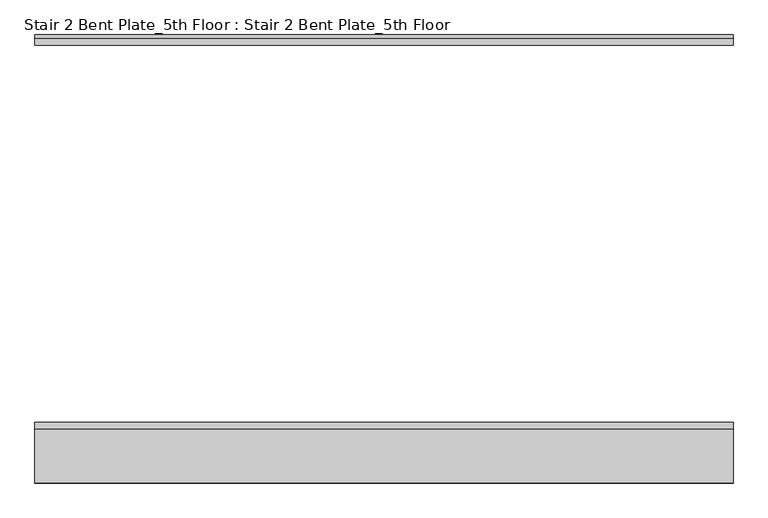
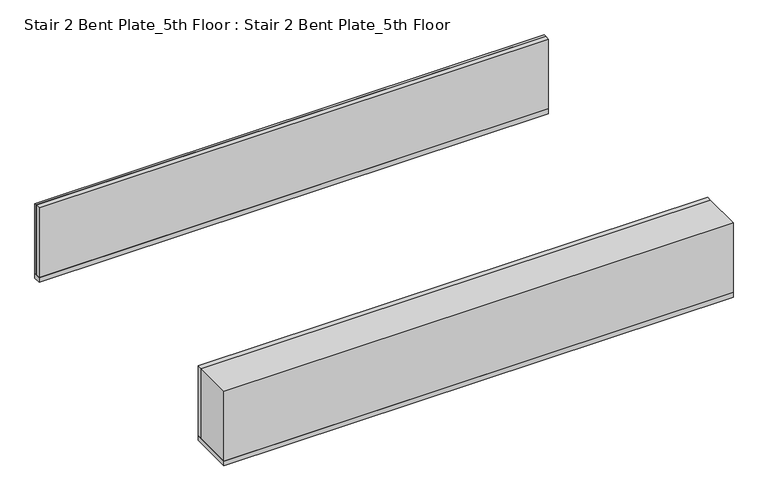
"""IFC4 building model written with IfcOpenShell, lengths in millimetres: proxy geometry, Stair 2 Bent Plate_5th Floor : Stair 2 Bent Plate_5th Floor."""

from ifc_helpers import new_model, si_unit, frame, origin, origin_with_axes, place, context, project, spatial, polyline, outline, extrude, source, transform, mapped, element, save


def stair_2_bent_plate_5th_floor_stair_2_bent_plate_5th_floor_55924f96(model_context):
    return source(origin(), model_context, "Body", "SweptSolid", [
        extrude(outline(polyline([(-247.65, -815.975), (-247.65, -714.375), (1066.8, -714.375), (1066.8, -815.975), (-247.65, -815.975)])), frame((0.0, 0.0, 12.7), z_axis=(0.0, 0.0, 1.0), x_axis=(1.0, 0.0, 0.0)), (0.0, 0.0, 1.0), 190.5),
        extrude(outline(polyline([(1066.8, 28.575), (1066.8, 22.225), (-247.65, 22.225), (-247.65, 28.575), (1066.8, 28.575)])), frame((0.0, 0.0, 12.7), z_axis=(0.0, 0.0, 1.0), x_axis=(1.0, 0.0, 0.0)), (0.0, 0.0, 1.0), 190.5),
        extrude(outline(polyline([(1066.8, -815.975), (-247.65, -815.975), (-247.65, -701.675), (1066.8, -701.675), (1066.8, -815.975)])), origin_with_axes(), (0.0, 0.0, 1.0), 12.7),
        extrude(outline(polyline([(1066.8, 9.525), (-247.65, 9.525), (-247.65, 28.575), (1066.8, 28.575), (1066.8, 9.525)])), origin_with_axes(), (0.0, 0.0, 1.0), 12.7),
        extrude(outline(polyline([(-247.65, -701.675), (1066.8, -701.675), (1066.8, -714.375), (-247.65, -714.375), (-247.65, -701.675)])), origin_with_axes(), (0.0, 0.0, 1.0), 203.2),
        extrude(outline(polyline([(1066.8, 9.525), (-247.65, 9.525), (-247.65, 22.225), (1066.8, 22.225), (1066.8, 9.525)])), origin_with_axes(), (0.0, 0.0, 1.0), 203.2),
    ])


if __name__ == "__main__":
    model = new_model("IFC4")
    model_context = context("Model", 3, world=origin())
    ifc_project = project(units=[si_unit("LENGTHUNIT", "METRE", prefix="MILLI")], contexts=[model_context])
    site = spatial("IfcSite", under=ifc_project)
    building = spatial("IfcBuilding", under=site)
    placement = place(None, origin())
    stair_2_bent_plate_5th_floor_stair_2_bent_plate_5th_floor_shape = stair_2_bent_plate_5th_floor_stair_2_bent_plate_5th_floor_55924f96(model_context)
    element("IfcBuildingElementProxy", 1, Name="Stair 2 Bent Plate_5th Floor : Stair 2 Bent Plate_5th Floor", ObjectType="Stair 2 Bent Plate_5th Floor : Stair 2 Bent Plate_5th Floor", at=placement, inside=building, context=model_context, shape_type="MappedRepresentation", body=[
        mapped(stair_2_bent_plate_5th_floor_stair_2_bent_plate_5th_floor_shape, transform((0.0, 0.0, 0.0), x_axis=(1.0, 0.0, 0.0), y_axis=(0.0, 1.0, 0.0), z_axis=(0.0, 0.0, 1.0))),
    ])
    save(model, "model.ifc")

# Revit data of these elements
# Element 1 (IfcBuildingElementProxy, "Stair 2 Bent Plate_5th Floor : Stair 2 Bent Plate_5th Floor")
#   Materials on its faces: "Concrete Infill"
# Materials
#   "Concrete Infill": class "Generic", colour RGB 0 255 0, transparency 0, Cost = 0
